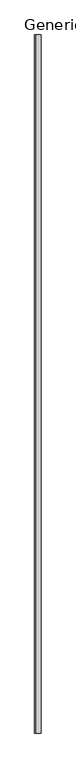
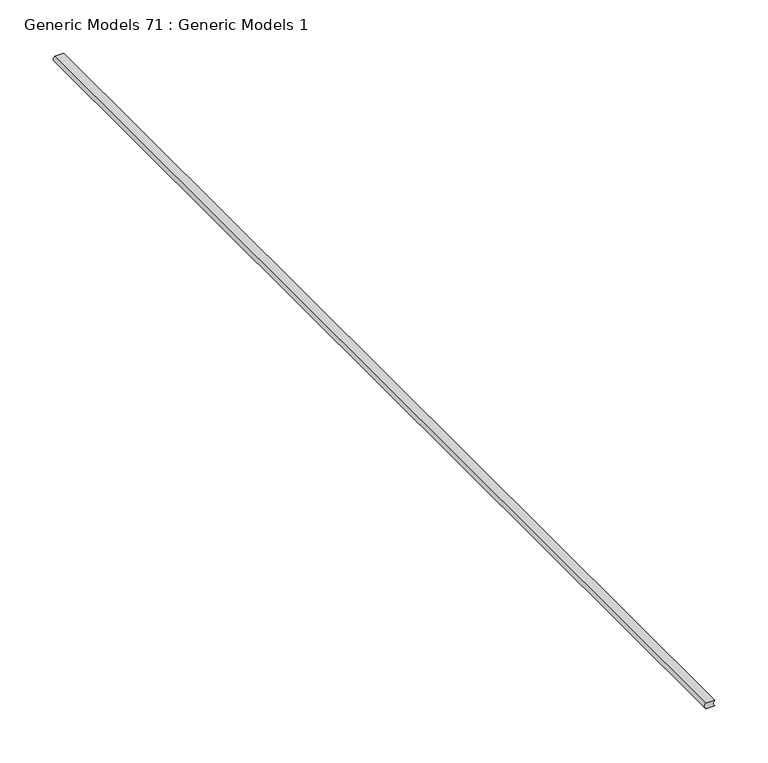
"""IFC4 building model written with IfcOpenShell, lengths in millimetres: proxy geometry, Generic Models 71 : Generic Models 1."""

from ifc_helpers import new_model, si_unit, point, frame, frame_2d, origin, place, context, project, spatial, polyline, circle_curve, trimmed, segment, composite_curve, outline, extrude, source, transform, mapped, element, save


def generic_models_71_generic_models_1_dfea5cc7(model_context):
    return source(origin(), model_context, "Body", "SweptSolid", [
        extrude(outline(composite_curve([segment(trimmed(circle_curve(frame_2d((31.025412, 51021.9897405)), 4.3100275), [point((27.850412, 51019.075))], [point((34.200412, 51019.075))], True, "CARTESIAN"), True, "CONTINUOUS"), segment(polyline([(34.200412, 51019.075), (34.200412, 51009.55)]), True, "CONTINUOUS"), segment(trimmed(circle_curve(frame_2d((31.025412, 51012.4647405)), 4.3100275), [point((34.200412, 51009.55))], [point((27.850412, 51009.55))], False, "CARTESIAN"), True, "CONTINUOUS"), segment(polyline([(27.850412, 51009.55), (27.850412, 51019.075)]), True, "CONTINUOUS")], self_intersect=False)), frame((0.0, 0.0, 0.0), z_axis=(0.0, 1.0, 0.0), x_axis=(0.0, 0.0, 1.0)), (0.0, 0.0, 1.0), 1219.2),
    ])


if __name__ == "__main__":
    model = new_model("IFC4")
    model_context = context("Model", 3, world=origin())
    ifc_project = project(units=[si_unit("LENGTHUNIT", "METRE", prefix="MILLI")], contexts=[model_context])
    site = spatial("IfcSite", under=ifc_project)
    building = spatial("IfcBuilding", under=site)
    placement = place(None, origin())
    generic_models_71_generic_models_1_shape = generic_models_71_generic_models_1_dfea5cc7(model_context)
    element("IfcBuildingElementProxy", 1, Name="Generic Models 71 : Generic Models 1", ObjectType="Generic Models 71 : Generic Models 1", at=placement, inside=building, context=model_context, shape_type="MappedRepresentation", body=[
        mapped(generic_models_71_generic_models_1_shape, transform((0.0, 0.0, 0.0), x_axis=(1.0, 0.0, 0.0), y_axis=(0.0, 1.0, 0.0), z_axis=(0.0, 0.0, 1.0))),
    ])
    save(model, "model.ifc")

# Revit data of these elements
# Element 1 (IfcBuildingElementProxy, "Generic Models 71 : Generic Models 1")
#   Materials on its faces: "ACOUSTICAL SEALANT"
# Materials
#   "ACOUSTICAL SEALANT": class "Unassigned", colour RGB 120 120 120, transparency 0, Cost = 0
